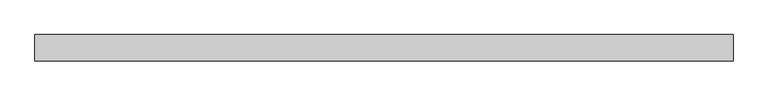
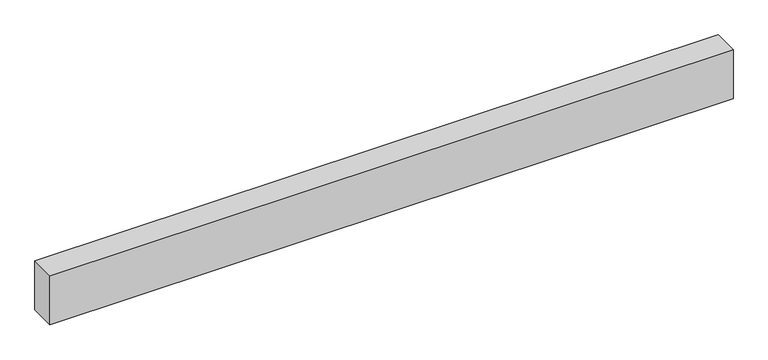
"""IFC4 building model written with IfcOpenShell, lengths in millimetres: beam geometry, Madeira de lei : Berço 6x12cm."""

import ifcopenshell
import ifcopenshell.guid

model = None  # the IFC model being written
_history = None  # IfcOwnerHistory: only IFC2X3 demands one
_inside = {}  # id of a spatial element -> (the spatial element, [elements in it])
_under = {}  # id of a project, library or spatial element -> (it, [spatial elements below it])
_declared = {}  # id of a project -> (the project, [libraries it declares])
_typed = {}  # id of a type object -> (the type object, [elements of that type])
_made_of = {}  # id of a material, layer set ... -> (it, [elements and type objects made of it])


def new_model(schema):
    """Start an empty IFC model of exactly this schema.

    Asked for "IFC4X3", IfcOpenShell would pick the latest addendum, in which some entities
    have other attributes; the version numbers below select the first issue.
    IFC2X3 requires an IfcOwnerHistory on every rooted entity: one is made here for all.
    """
    global model, _history
    if schema == "IFC4X3":
        model = ifcopenshell.file(schema_version=(4, 3, 0, 0))
    else:
        model = ifcopenshell.file(schema=schema)
    _inside.clear()
    _under.clear()
    _declared.clear()
    _typed.clear()
    _made_of.clear()
    _history = None
    if model.schema == "IFC2X3":
        org = make("IfcOrganization", Name="unknown")
        user = make(
            "IfcPersonAndOrganization",
            ThePerson=make("IfcPerson", FamilyName="unknown"),
            TheOrganization=org,
        )
        app = make(
            "IfcApplication",
            ApplicationDeveloper=org,
            Version="unknown",
            ApplicationFullName="unknown",
            ApplicationIdentifier="unknown",
        )
        _history = make(
            "IfcOwnerHistory",
            OwningUser=user,
            OwningApplication=app,
            ChangeAction="ADDED",
            CreationDate=0,
        )
    return model


def make(cls, **values):
    """One entity of the class cls with the attributes given. An attribute that is None is left unset."""
    return model.create_entity(
        cls, **{name: value for name, value in values.items() if value is not None}
    )


def rooted(cls, **values):
    """An entity with a GlobalId (a new one), such as an element, a storey or a relation."""
    return make(cls, GlobalId=ifcopenshell.guid.new(), OwnerHistory=_history, **values)


def si_unit(unit_type, name, prefix=None):
    """IfcSIUnit, for example si_unit("LENGTHUNIT", "METRE", prefix="MILLI")."""
    return make("IfcSIUnit", UnitType=unit_type, Prefix=prefix, Name=name)


def assignment(units):
    """IfcUnitAssignment: the units of a project."""
    return None if units is None else make("IfcUnitAssignment", Units=units)


def point(xyz):
    """IfcCartesianPoint."""
    return None if xyz is None else make("IfcCartesianPoint", Coordinates=xyz)


def direction(xyz):
    """IfcDirection."""
    return None if xyz is None else make("IfcDirection", DirectionRatios=xyz)


def frame(location, z_axis=None, x_axis=None):
    """IfcAxis2Placement3D, a coordinate frame: its origin and axes. An axis left out is left unset."""
    return make(
        "IfcAxis2Placement3D",
        Location=point(location),
        Axis=direction(z_axis),
        RefDirection=direction(x_axis),
    )


def origin():
    """The frame at (0, 0, 0) with its axes left unset."""
    return frame((0.0, 0.0, 0.0))


def place(relative_to, where):
    """IfcLocalPlacement: puts the frame where relative to a parent placement (None: the world)."""
    return make(
        "IfcLocalPlacement", PlacementRelTo=relative_to, RelativePlacement=where
    )


def context(
    kind, dimensions, precision=None, world=None, true_north=None, identifier=None
):
    """IfcGeometricRepresentationContext, for example the 3D "Model" context."""
    return make(
        "IfcGeometricRepresentationContext",
        ContextIdentifier=identifier,
        ContextType=kind,
        CoordinateSpaceDimension=dimensions,
        Precision=precision,
        WorldCoordinateSystem=world,
        TrueNorth=true_north,
    )


def project(units=None, contexts=None):
    """IfcProject with its units and contexts."""
    return rooted(
        "IfcProject",
        Name="project",
        RepresentationContexts=contexts,
        UnitsInContext=assignment(units),
    )


def spatial(cls, under=None, at=None, **own):
    """A site, building, storey or space (cls), placed at a placement, below another one or the project."""
    s = rooted(cls, ObjectPlacement=at, **own)
    if under is not None:
        _under.setdefault(under.id(), (under, []))[1].append(s)
    return s


def polyline(points):
    """IfcPolyline through the points."""
    return make("IfcPolyline", Points=[point(p) for p in points])


def outline(outer, holes=None, kind="AREA"):
    """IfcArbitraryClosedProfileDef: a profile drawn as a closed curve; with holes, ...WithVoids."""
    if holes is None:
        return make("IfcArbitraryClosedProfileDef", ProfileType=kind, OuterCurve=outer)
    return make(
        "IfcArbitraryProfileDefWithVoids",
        ProfileType=kind,
        OuterCurve=outer,
        InnerCurves=holes,
    )


def extrude(swept, where, along, depth):
    """IfcExtrudedAreaSolid: the profile swept, set in the frame where, extruded along a direction by depth."""
    return make(
        "IfcExtrudedAreaSolid",
        SweptArea=swept,
        Position=where,
        ExtrudedDirection=direction(along),
        Depth=depth,
    )


def shape(context_of_items, identifier, shape_type, items):
    """IfcShapeRepresentation: the items that make up one representation, for example the "Body"."""
    return make(
        "IfcShapeRepresentation",
        ContextOfItems=context_of_items,
        RepresentationIdentifier=identifier,
        RepresentationType=shape_type,
        Items=items,
    )


def source(mapping_origin, context_of_items, identifier, shape_type, items):
    """IfcRepresentationMap: a shape defined once, which mapped items show again and again."""
    return make(
        "IfcRepresentationMap",
        MappingOrigin=mapping_origin,
        MappedRepresentation=shape(context_of_items, identifier, shape_type, items),
    )


def transform(
    local_origin,
    x_axis=None,
    y_axis=None,
    z_axis=None,
    scale=None,
    scale2=None,
    scale3=None,
    uniform=True,
):
    """IfcCartesianTransformationOperator3D, or its non-uniform kind. x_axis, y_axis, z_axis: its Axis1, 2, 3."""
    if uniform:
        return make(
            "IfcCartesianTransformationOperator3D",
            Axis1=direction(x_axis),
            Axis2=direction(y_axis),
            LocalOrigin=point(local_origin),
            Scale=scale,
            Axis3=direction(z_axis),
        )
    return make(
        "IfcCartesianTransformationOperator3DnonUniform",
        Axis1=direction(x_axis),
        Axis2=direction(y_axis),
        LocalOrigin=point(local_origin),
        Scale=scale,
        Axis3=direction(z_axis),
        Scale2=scale2,
        Scale3=scale3,
    )


def mapped(mapping_source, mapping_target):
    """IfcMappedItem: shows the shape of a source again, moved by a transform."""
    return make(
        "IfcMappedItem", MappingSource=mapping_source, MappingTarget=mapping_target
    )


def made_of(thing, what):
    """Note that an element or type object is made of a material, layer set ...; save() writes the relation."""
    if what is not None:
        _made_of.setdefault(what.id(), (what, []))[1].append(thing)
    return thing


def element(
    cls,
    number,
    at=None,
    inside=None,
    cuts=None,
    type_object=None,
    material=None,
    context=None,
    identifier="Body",
    shape_type=None,
    held_by="IfcProductDefinitionShape",
    body=None,
    shapes=None,
    **own,
):
    """One element of the class cls, such as IfcWall. Its Tag is "e" and its number.

    at: its placement. inside: the storey or other place that contains it. cuts: it is an
    opening in that element (IfcRelVoidsElement). A single representation is given by context,
    identifier, shape_type and body (its items); several are given by shapes. held_by: the class
    of the entity that holds the representations. save() writes the other relations.
    """
    e = rooted(cls, Tag="e%d" % number, ObjectPlacement=at, **own)
    if body is not None:
        shapes = [shape(context, identifier, shape_type, body)]
    if shapes is not None:
        e.Representation = make(held_by, Representations=shapes)
    if inside is not None:
        _inside.setdefault(inside.id(), (inside, []))[1].append(e)
    if cuts is not None:
        rooted(
            "IfcRelVoidsElement", RelatingBuildingElement=cuts, RelatedOpeningElement=e
        )
    if type_object is not None:
        _typed.setdefault(type_object.id(), (type_object, []))[1].append(e)
    return made_of(e, material)


def aggregate(whole, parts):
    """IfcRelAggregates: a whole, such as a stair, and the parts it consists of."""
    return rooted("IfcRelAggregates", RelatingObject=whole, RelatedObjects=parts)


def save(model, path):
    """Write the relations noted so far, then the file.

    IfcRelAggregates (storeys below a building ...), IfcRelContainedInSpatialStructure (elements
    in a storey), IfcRelDefinesByType, IfcRelAssociatesMaterial and IfcRelDeclares: one each for
    every whole, place, type object, material and project.
    """
    for whole, parts in _under.values():
        aggregate(whole, parts)
    for where, things in _inside.values():
        rooted(
            "IfcRelContainedInSpatialStructure",
            RelatedElements=things,
            RelatingStructure=where,
        )
    for kind, things in _typed.values():
        rooted("IfcRelDefinesByType", RelatedObjects=things, RelatingType=kind)
    for what, things in _made_of.values():
        rooted("IfcRelAssociatesMaterial", RelatedObjects=things, RelatingMaterial=what)
    for by, libraries in _declared.values():
        rooted("IfcRelDeclares", RelatingContext=by, RelatedDefinitions=libraries)
    model.write(path)


def beam_531541e1(model_context):
    return source(origin(), model_context, "Body", "SweptSolid", [
        extrude(outline(polyline([(789.5608169, 30.0), (789.5608169, -30.0), (-789.5608169, -30.0), (-789.5608169, 30.0), (789.5608169, 30.0)])), frame((0.0, 0.0, -60.0), z_axis=(0.0, 0.0, 1.0), x_axis=(1.0, 0.0, 0.0)), (0.0, 0.0, 1.0), 120.0),
    ])


if __name__ == "__main__":
    model = new_model("IFC4")
    model_context = context("Model", 3, world=origin())
    ifc_project = project(units=[si_unit("LENGTHUNIT", "METRE", prefix="MILLI")], contexts=[model_context])
    site = spatial("IfcSite", under=ifc_project)
    building = spatial("IfcBuilding", under=site)
    placement = place(None, origin())
    beam_shape = beam_531541e1(model_context)
    element("IfcBeam", 1, ObjectType="Madeira de lei : Berço 6x12cm", at=placement, inside=building, context=model_context, shape_type="MappedRepresentation", body=[
        mapped(beam_shape, transform((0.0, 0.0, 0.0), x_axis=(1.0, 0.0, 0.0), y_axis=(0.0, 1.0, 0.0), z_axis=(0.0, 0.0, 1.0))),
    ])
    save(model, "model.ifc")

# Revit data of these elements
# Type "Madeira de lei : Berço 6x12cm"
#   A = 0.02 m²
#   Length [instance default] = 1.524 m
#   b = 0.06 m
#   d = 0.12 m
#   Structural Material [instance default] = none
#   Assembly Code = ""
# Element 1 (IfcBeam, "Madeira de lei : Berço 6x12cm")
#   Structural Material = .MADEIRAMENTO
#   Materials on its faces: ".MADEIRAMENTO"
# Materials
#   ".MADEIRAMENTO": class ".CC_MADEIRAS", colour RGB 212 179 113, transparency 0, Cost = 0
